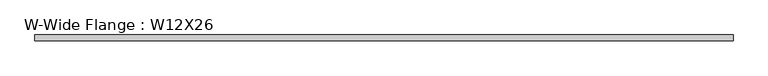
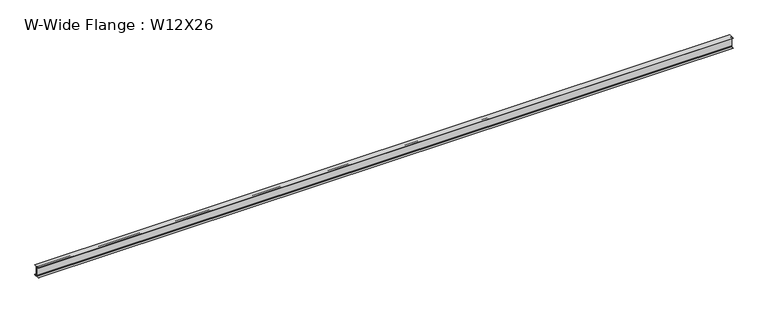
"""IFC4 building model written with IfcOpenShell, lengths in millimetres: beam geometry, W-Wide Flange : W12X26."""

from ifc_helpers import new_model, si_unit, point, frame, frame_2d, origin, place, context, project, spatial, polyline, circle_curve, trimmed, segment, composite_curve, outline, extrude, source, transform, mapped, element, save


def w_wide_flange_w12x26_d132d5fd(model_context):
    return source(origin(), model_context, "Body", "SweptSolid", [
        extrude(outline(composite_curve([segment(polyline([(82.4011719, -145.5539063), (82.4011719, -155.178125), (-82.4011719, -155.178125), (-82.4011719, -145.5539063), (-20.2902344, -145.5539063)]), True, "CONTINUOUS"), segment(trimmed(circle_curve(frame_2d((-20.2902344, -128.190625)), 17.3632812), [point((-20.2902344, -145.5539063))], [point((-2.9269531, -128.190625))], True, "CARTESIAN"), True, "CONTINUOUS"), segment(polyline([(-2.9269531, -128.190625), (-2.9269531, 128.190625)]), True, "CONTINUOUS"), segment(trimmed(circle_curve(frame_2d((-20.2902344, 128.190625)), 17.3632812), [point((-2.9269531, 128.190625))], [point((-20.2902344, 145.5539062))], True, "CARTESIAN"), True, "CONTINUOUS"), segment(polyline([(-20.2902344, 145.5539062), (-82.4011719, 145.5539062), (-82.4011719, 155.178125), (82.4011719, 155.178125), (82.4011719, 145.5539062), (20.2902344, 145.5539062)]), True, "CONTINUOUS"), segment(trimmed(circle_curve(frame_2d((20.2902344, 128.190625)), 17.3632812), [point((20.2902344, 145.5539062))], [point((2.9269531, 128.190625))], True, "CARTESIAN"), True, "CONTINUOUS"), segment(polyline([(2.9269531, 128.190625), (2.9269531, -128.190625)]), True, "CONTINUOUS"), segment(trimmed(circle_curve(frame_2d((20.2902344, -128.190625)), 17.3632812), [point((2.9269531, -128.190625))], [point((20.2902344, -145.5539063))], True, "CARTESIAN"), True, "CONTINUOUS"), segment(polyline([(20.2902344, -145.5539063), (82.4011719, -145.5539063)]), True, "CONTINUOUS")], self_intersect=False)), frame((-10136.0386719, 0.0, 0.0), z_axis=(1.0, 0.0, 0.0), x_axis=(0.0, 1.0, 0.0)), (0.0, 0.0, 1.0), 20080.1386719),
    ])


if __name__ == "__main__":
    model = new_model("IFC4")
    model_context = context("Model", 3, world=origin())
    ifc_project = project(units=[si_unit("LENGTHUNIT", "METRE", prefix="MILLI")], contexts=[model_context])
    site = spatial("IfcSite", under=ifc_project)
    building = spatial("IfcBuilding", under=site)
    placement = place(None, origin())
    w_wide_flange_w12x26_shape = w_wide_flange_w12x26_d132d5fd(model_context)
    element("IfcBeam", 1, ObjectType="W-Wide Flange : W12X26", at=placement, inside=building, context=model_context, shape_type="MappedRepresentation", body=[
        mapped(w_wide_flange_w12x26_shape, transform((0.0, 0.0, 0.0), x_axis=(1.0, 0.0, 0.0), y_axis=(0.0, 1.0, 0.0), z_axis=(0.0, 0.0, 1.0))),
    ])
    save(model, "model.ifc")

# Revit data of these elements
# Type "W-Wide Flange : W12X26"
#   Assembly Code = "B10"
#   W = 26
#   Length [instance default] = 5' - 0"
#   bf = 0' - 6 125/256"
#   d = 1' - 0 7/32"
#   k = 0' - 1 1/16"
#   k2 = 0' - 0 175/256"
#   tf = 0' - 0 97/256"
#   tw = 0' - 0 59/256"
#   A = 0.053125 SF
#   Structural Material [instance default] = none
# Element 1 (IfcBeam, "W-Wide Flange : W12X26")
#   Structural Material = Dark metal
#   Materials on its faces: "Dark metal"
# Materials
#   "Dark metal": class "Generic", colour RGB 44 29 29, transparency 0, Cost = 0
